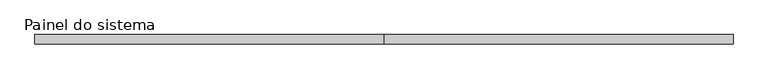
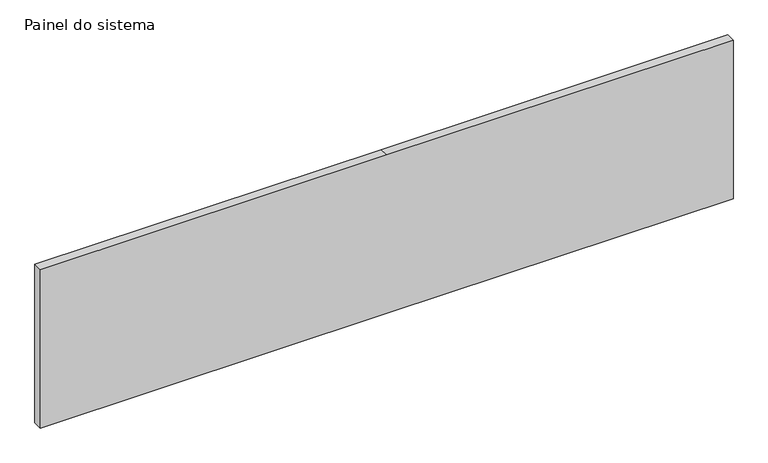
"""IFC4 building model written with IfcOpenShell, lengths in millimetres: plate geometry, Painel do sistema : Envidraçado."""

import ifcopenshell
import ifcopenshell.guid

model = None  # the IFC model being written
_history = None  # IfcOwnerHistory: only IFC2X3 demands one
_inside = {}  # id of a spatial element -> (the spatial element, [elements in it])
_under = {}  # id of a project, library or spatial element -> (it, [spatial elements below it])
_declared = {}  # id of a project -> (the project, [libraries it declares])
_typed = {}  # id of a type object -> (the type object, [elements of that type])
_made_of = {}  # id of a material, layer set ... -> (it, [elements and type objects made of it])


def new_model(schema):
    """Start an empty IFC model of exactly this schema.

    Asked for "IFC4X3", IfcOpenShell would pick the latest addendum, in which some entities
    have other attributes; the version numbers below select the first issue.
    IFC2X3 requires an IfcOwnerHistory on every rooted entity: one is made here for all.
    """
    global model, _history
    if schema == "IFC4X3":
        model = ifcopenshell.file(schema_version=(4, 3, 0, 0))
    else:
        model = ifcopenshell.file(schema=schema)
    _inside.clear()
    _under.clear()
    _declared.clear()
    _typed.clear()
    _made_of.clear()
    _history = None
    if model.schema == "IFC2X3":
        org = make("IfcOrganization", Name="unknown")
        user = make(
            "IfcPersonAndOrganization",
            ThePerson=make("IfcPerson", FamilyName="unknown"),
            TheOrganization=org,
        )
        app = make(
            "IfcApplication",
            ApplicationDeveloper=org,
            Version="unknown",
            ApplicationFullName="unknown",
            ApplicationIdentifier="unknown",
        )
        _history = make(
            "IfcOwnerHistory",
            OwningUser=user,
            OwningApplication=app,
            ChangeAction="ADDED",
            CreationDate=0,
        )
    return model


def make(cls, **values):
    """One entity of the class cls with the attributes given. An attribute that is None is left unset."""
    return model.create_entity(
        cls, **{name: value for name, value in values.items() if value is not None}
    )


def rooted(cls, **values):
    """An entity with a GlobalId (a new one), such as an element, a storey or a relation."""
    return make(cls, GlobalId=ifcopenshell.guid.new(), OwnerHistory=_history, **values)


def si_unit(unit_type, name, prefix=None):
    """IfcSIUnit, for example si_unit("LENGTHUNIT", "METRE", prefix="MILLI")."""
    return make("IfcSIUnit", UnitType=unit_type, Prefix=prefix, Name=name)


def assignment(units):
    """IfcUnitAssignment: the units of a project."""
    return None if units is None else make("IfcUnitAssignment", Units=units)


def point(xyz):
    """IfcCartesianPoint."""
    return None if xyz is None else make("IfcCartesianPoint", Coordinates=xyz)


def direction(xyz):
    """IfcDirection."""
    return None if xyz is None else make("IfcDirection", DirectionRatios=xyz)


def frame(location, z_axis=None, x_axis=None):
    """IfcAxis2Placement3D, a coordinate frame: its origin and axes. An axis left out is left unset."""
    return make(
        "IfcAxis2Placement3D",
        Location=point(location),
        Axis=direction(z_axis),
        RefDirection=direction(x_axis),
    )


def origin():
    """The frame at (0, 0, 0) with its axes left unset."""
    return frame((0.0, 0.0, 0.0))


def place(relative_to, where):
    """IfcLocalPlacement: puts the frame where relative to a parent placement (None: the world)."""
    return make(
        "IfcLocalPlacement", PlacementRelTo=relative_to, RelativePlacement=where
    )


def context(
    kind, dimensions, precision=None, world=None, true_north=None, identifier=None
):
    """IfcGeometricRepresentationContext, for example the 3D "Model" context."""
    return make(
        "IfcGeometricRepresentationContext",
        ContextIdentifier=identifier,
        ContextType=kind,
        CoordinateSpaceDimension=dimensions,
        Precision=precision,
        WorldCoordinateSystem=world,
        TrueNorth=true_north,
    )


def project(units=None, contexts=None):
    """IfcProject with its units and contexts."""
    return rooted(
        "IfcProject",
        Name="project",
        RepresentationContexts=contexts,
        UnitsInContext=assignment(units),
    )


def spatial(cls, under=None, at=None, **own):
    """A site, building, storey or space (cls), placed at a placement, below another one or the project."""
    s = rooted(cls, ObjectPlacement=at, **own)
    if under is not None:
        _under.setdefault(under.id(), (under, []))[1].append(s)
    return s


def polyline(points):
    """IfcPolyline through the points."""
    return make("IfcPolyline", Points=[point(p) for p in points])


def outline(outer, holes=None, kind="AREA"):
    """IfcArbitraryClosedProfileDef: a profile drawn as a closed curve; with holes, ...WithVoids."""
    if holes is None:
        return make("IfcArbitraryClosedProfileDef", ProfileType=kind, OuterCurve=outer)
    return make(
        "IfcArbitraryProfileDefWithVoids",
        ProfileType=kind,
        OuterCurve=outer,
        InnerCurves=holes,
    )


def extrude(swept, where, along, depth):
    """IfcExtrudedAreaSolid: the profile swept, set in the frame where, extruded along a direction by depth."""
    return make(
        "IfcExtrudedAreaSolid",
        SweptArea=swept,
        Position=where,
        ExtrudedDirection=direction(along),
        Depth=depth,
    )


def shape(context_of_items, identifier, shape_type, items):
    """IfcShapeRepresentation: the items that make up one representation, for example the "Body"."""
    return make(
        "IfcShapeRepresentation",
        ContextOfItems=context_of_items,
        RepresentationIdentifier=identifier,
        RepresentationType=shape_type,
        Items=items,
    )


def source(mapping_origin, context_of_items, identifier, shape_type, items):
    """IfcRepresentationMap: a shape defined once, which mapped items show again and again."""
    return make(
        "IfcRepresentationMap",
        MappingOrigin=mapping_origin,
        MappedRepresentation=shape(context_of_items, identifier, shape_type, items),
    )


def transform(
    local_origin,
    x_axis=None,
    y_axis=None,
    z_axis=None,
    scale=None,
    scale2=None,
    scale3=None,
    uniform=True,
):
    """IfcCartesianTransformationOperator3D, or its non-uniform kind. x_axis, y_axis, z_axis: its Axis1, 2, 3."""
    if uniform:
        return make(
            "IfcCartesianTransformationOperator3D",
            Axis1=direction(x_axis),
            Axis2=direction(y_axis),
            LocalOrigin=point(local_origin),
            Scale=scale,
            Axis3=direction(z_axis),
        )
    return make(
        "IfcCartesianTransformationOperator3DnonUniform",
        Axis1=direction(x_axis),
        Axis2=direction(y_axis),
        LocalOrigin=point(local_origin),
        Scale=scale,
        Axis3=direction(z_axis),
        Scale2=scale2,
        Scale3=scale3,
    )


def mapped(mapping_source, mapping_target):
    """IfcMappedItem: shows the shape of a source again, moved by a transform."""
    return make(
        "IfcMappedItem", MappingSource=mapping_source, MappingTarget=mapping_target
    )


def made_of(thing, what):
    """Note that an element or type object is made of a material, layer set ...; save() writes the relation."""
    if what is not None:
        _made_of.setdefault(what.id(), (what, []))[1].append(thing)
    return thing


def element(
    cls,
    number,
    at=None,
    inside=None,
    cuts=None,
    type_object=None,
    material=None,
    context=None,
    identifier="Body",
    shape_type=None,
    held_by="IfcProductDefinitionShape",
    body=None,
    shapes=None,
    **own,
):
    """One element of the class cls, such as IfcWall. Its Tag is "e" and its number.

    at: its placement. inside: the storey or other place that contains it. cuts: it is an
    opening in that element (IfcRelVoidsElement). A single representation is given by context,
    identifier, shape_type and body (its items); several are given by shapes. held_by: the class
    of the entity that holds the representations. save() writes the other relations.
    """
    e = rooted(cls, Tag="e%d" % number, ObjectPlacement=at, **own)
    if body is not None:
        shapes = [shape(context, identifier, shape_type, body)]
    if shapes is not None:
        e.Representation = make(held_by, Representations=shapes)
    if inside is not None:
        _inside.setdefault(inside.id(), (inside, []))[1].append(e)
    if cuts is not None:
        rooted(
            "IfcRelVoidsElement", RelatingBuildingElement=cuts, RelatedOpeningElement=e
        )
    if type_object is not None:
        _typed.setdefault(type_object.id(), (type_object, []))[1].append(e)
    return made_of(e, material)


def aggregate(whole, parts):
    """IfcRelAggregates: a whole, such as a stair, and the parts it consists of."""
    return rooted("IfcRelAggregates", RelatingObject=whole, RelatedObjects=parts)


def save(model, path):
    """Write the relations noted so far, then the file.

    IfcRelAggregates (storeys below a building ...), IfcRelContainedInSpatialStructure (elements
    in a storey), IfcRelDefinesByType, IfcRelAssociatesMaterial and IfcRelDeclares: one each for
    every whole, place, type object, material and project.
    """
    for whole, parts in _under.values():
        aggregate(whole, parts)
    for where, things in _inside.values():
        rooted(
            "IfcRelContainedInSpatialStructure",
            RelatedElements=things,
            RelatingStructure=where,
        )
    for kind, things in _typed.values():
        rooted("IfcRelDefinesByType", RelatedObjects=things, RelatingType=kind)
    for what, things in _made_of.values():
        rooted("IfcRelAssociatesMaterial", RelatedObjects=things, RelatingMaterial=what)
    for by, libraries in _declared.values():
        rooted("IfcRelDeclares", RelatingContext=by, RelatedDefinitions=libraries)
    model.write(path)


def painel_do_sistema_b648e332(model_context):
    return source(origin(), model_context, "Body", "SweptSolid", [
        extrude(outline(polyline([(0.0, -931.0166666), (0.0, 0.0), (0.0, 931.0166666), (450.0, 931.0166666), (450.0, 0.0), (450.0, -931.0166666), (0.0, -931.0166666)])), frame((0.0, 24.5, 0.0), z_axis=(0.0, 1.0, 0.0), x_axis=(0.0, 0.0, 1.0)), (0.0, 0.0, 1.0), 25.0),
    ])


if __name__ == "__main__":
    model = new_model("IFC4")
    model_context = context("Model", 3, world=origin())
    ifc_project = project(units=[si_unit("LENGTHUNIT", "METRE", prefix="MILLI")], contexts=[model_context])
    site = spatial("IfcSite", under=ifc_project)
    building = spatial("IfcBuilding", under=site)
    placement = place(None, origin())
    painel_do_sistema_shape = painel_do_sistema_b648e332(model_context)
    element("IfcPlate", 1, ObjectType="Painel do sistema : Envidraçado", at=placement, inside=building, context=model_context, shape_type="MappedRepresentation", body=[
        mapped(painel_do_sistema_shape, transform((0.0, 0.0, 0.0), x_axis=(1.0, 0.0, 0.0), y_axis=(0.0, 1.0, 0.0), z_axis=(0.0, 0.0, 1.0))),
    ])
    save(model, "model.ifc")

# Revit data of these elements
# Type "Painel do sistema : Envidraçado"
#   Construction Type Id = "GSP4R"
#   Analytic Construction = "Vidraça única Pilkington 1/8 pol"
#   Visual Light Transmittance = 0.9
#   Solar Heat Gain Coefficient = 0.86
#   Heat Transfer Coefficient (U) = 6.7069 W/(m²·K)
# Element 1 (IfcPlate, "Painel do sistema : Envidraçado")
#   Materials on its faces: ".VIDRO GENÉRICO"
# Materials
#   ".VIDRO GENÉRICO": class ".CC_VIDRO", colour RGB 0 128 192, transparency 0.9, Description = "Vidro comum", Cost = 0
